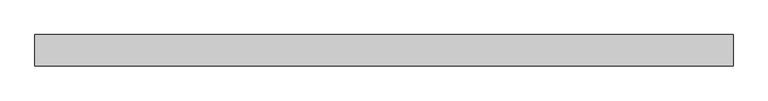
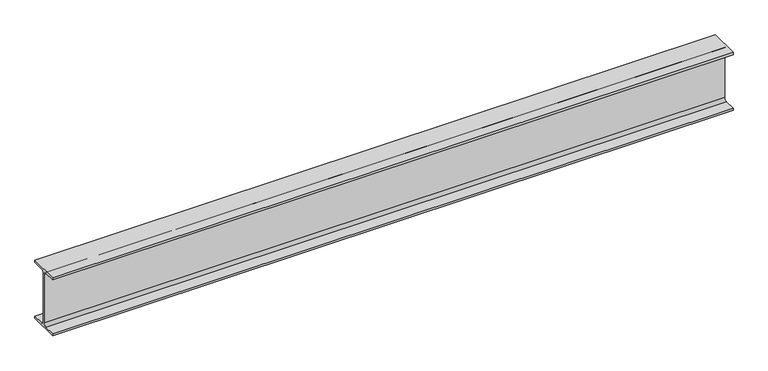
"""IFC4 building model written with IfcOpenShell, lengths in millimetres: beam geometry, 0912_Steel Framing_H-KSD3502 : H_SB_ASB_H-250x125x6x9."""

from ifc_helpers import new_model, si_unit, point, frame, frame_2d, origin, place, context, project, spatial, polyline, circle_curve, trimmed, segment, composite_curve, outline, extrude, source, transform, mapped, element, save


def beam_0840c79e(model_context):
    return source(origin(), model_context, "Body", "SweptSolid", [
        extrude(outline(composite_curve([segment(polyline([(62.5, -116.0), (62.5, -125.0), (-62.5, -125.0), (-62.5, -116.0), (-15.0, -116.0)]), True, "CONTINUOUS"), segment(trimmed(circle_curve(frame_2d((-15.0, -104.0)), 12.0), [point((-15.0, -116.0))], [point((-3.0, -104.0))], True, "CARTESIAN"), True, "CONTINUOUS"), segment(polyline([(-3.0, -104.0), (-3.0, 104.0)]), True, "CONTINUOUS"), segment(trimmed(circle_curve(frame_2d((-15.0, 104.0)), 12.0), [point((-3.0, 104.0))], [point((-15.0, 116.0))], True, "CARTESIAN"), True, "CONTINUOUS"), segment(polyline([(-15.0, 116.0), (-62.5, 116.0), (-62.5, 125.0), (62.5, 125.0), (62.5, 116.0), (15.0, 116.0)]), True, "CONTINUOUS"), segment(trimmed(circle_curve(frame_2d((15.0, 104.0)), 12.0), [point((15.0, 116.0))], [point((3.0, 104.0))], True, "CARTESIAN"), True, "CONTINUOUS"), segment(polyline([(3.0, 104.0), (3.0, -104.0)]), True, "CONTINUOUS"), segment(trimmed(circle_curve(frame_2d((15.0, -104.0)), 12.0), [point((3.0, -104.0))], [point((15.0, -116.0))], True, "CARTESIAN"), True, "CONTINUOUS"), segment(polyline([(15.0, -116.0), (62.5, -116.0)]), True, "CONTINUOUS")], self_intersect=False)), frame((-1387.3, 0.0, 0.0), z_axis=(1.0, 0.0, 0.0), x_axis=(0.0, 1.0, 0.0)), (0.0, 0.0, 1.0), 2774.6),
    ])


if __name__ == "__main__":
    model = new_model("IFC4")
    model_context = context("Model", 3, world=origin())
    ifc_project = project(units=[si_unit("LENGTHUNIT", "METRE", prefix="MILLI")], contexts=[model_context])
    site = spatial("IfcSite", under=ifc_project)
    building = spatial("IfcBuilding", under=site)
    placement = place(None, origin())
    beam_shape = beam_0840c79e(model_context)
    element("IfcBeam", 1, ObjectType="0912_Steel Framing_H-KSD3502 : H_SB_ASB_H-250x125x6x9", at=placement, inside=building, context=model_context, shape_type="MappedRepresentation", body=[
        mapped(beam_shape, transform((0.0, 0.0, 0.0), x_axis=(1.0, 0.0, 0.0), y_axis=(0.0, 1.0, 0.0), z_axis=(0.0, 0.0, 1.0))),
    ])
    save(model, "model.ifc")

# Revit data of these elements
# Type "0912_Steel Framing_H-KSD3502 : H_SB_ASB_H-250x125x6x9"
#   H_WM Code_1 = "S01AA003-00001 | Main Steel Structure Fabrication Work | Shelter/Building | Light Steel - Standard (30KG/M>Weight) | Material: (   )"
#   H_WM Code_2 = "S03AA029-00001 | Main Steel Structure Erection Work | Shelter/Building | Light Steel (30KG/M>Weight) | Material: (   )"
#   H_WM Code_3 = "S01AA010-00001 | Main Steel Structure Fabrication Work | Shelter/Building | Steel Painting/Coating | for Non-Fireproofed Steel Surface, Surface Preparation, Primer, Second & Final Coat | Material: (   )"
#   H_Q'ty Cal Type Tag = "SB-Q2"
#   Width = 12.5 cm
#   Web Thickness = 0.6 cm
#   Web Fillet = 1.2 cm
#   Warping Constant = 42539.8 cm⁶
#   W = 0
#   Torsional Moment of Inertia = 7.8102 cm⁴
#   Section Area = 37.66 cm²
#   Plastic Modulus weak axis = 73.1 cm³
#   Plastic Modulus strong axis = 366.0 cm³
#   Perimeter = 0.97 m²/m
#   Nominal Weight = 29.60 kgf/m
#   Moment of Inertia weak axis = 294.00 cm⁴
#   Moment of Inertia strong axis = 4050.00 cm⁴
#   Height = 25.0 cm
#   Flange Thickness = 0.9 cm
#   Elastic Modulus weak axis = 47.0 cm³
#   Elastic Modulus strong axis = 324.0 cm³
#   Centroid Vertical = 12.5 cm
#   Centroid Horizontal = 6.25 cm
#   Ix = 40500000
#   Length [instance default] = 1.5240 m
#   Zx = 366000
#   b = 0.1250 m
#   h = 0.2500 m
#   r = 0.0120 m
#   s = 0.0060 m
#   t = 0.0090 m
#   A = 0.003766 m²
#   Structural Material [instance default] = Steel, 45-345
#   Assembly Code = ""
# Element 1 (IfcBeam, "0912_Steel Framing_H-KSD3502 : H_SB_ASB_H-250x125x6x9")
#   Structural Material = none
# Materials
#   "Steel, 45-345": class "Metal", colour RGB 189 187 185, transparency 0, Description = "Steel 345 MPa", Cost = 0
